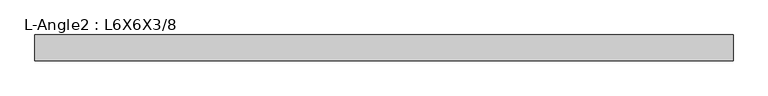
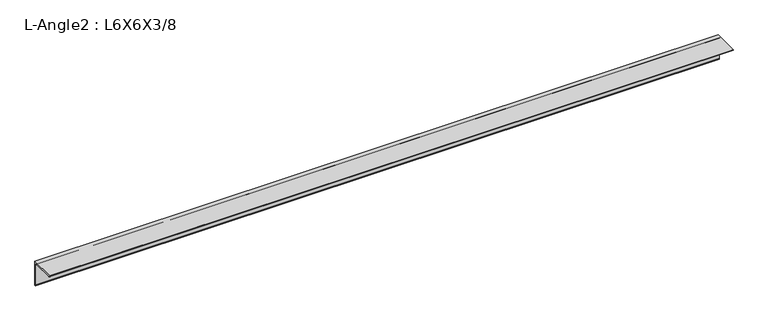
"""IFC4 building model written with IfcOpenShell, lengths in millimetres: member geometry, L-Angle2 : L6X6X3/8."""

from ifc_helpers import new_model, si_unit, point, frame, frame_2d, origin, place, context, project, spatial, polyline, circle_curve, trimmed, segment, composite_curve, outline, extrude, source, transform, mapped, element, save


def l_angle2_l6x6x3_8_670392f0(model_context):
    return source(origin(), model_context, "Body", "SweptSolid", [
        extrude(outline(composite_curve([segment(polyline([(41.148, 41.148), (41.148, -111.252)]), True, "CONTINUOUS"), segment(trimmed(circle_curve(frame_2d((41.148, -101.727)), 9.525), [point((41.148, -111.252))], [point((31.623, -101.727))], False, "CARTESIAN"), True, "CONTINUOUS"), segment(polyline([(31.623, -101.727), (31.623, 22.098)]), True, "CONTINUOUS"), segment(trimmed(circle_curve(frame_2d((22.098, 22.098)), 9.525), [point((31.623, 22.098))], [point((22.098, 31.623))], True, "CARTESIAN"), True, "CONTINUOUS"), segment(polyline([(22.098, 31.623), (-101.727, 31.623)]), True, "CONTINUOUS"), segment(trimmed(circle_curve(frame_2d((-101.727, 41.148)), 9.525), [point((-101.727, 31.623))], [point((-111.252, 41.148))], False, "CARTESIAN"), True, "CONTINUOUS"), segment(polyline([(-111.252, 41.148), (41.148, 41.148)]), True, "CONTINUOUS")], self_intersect=False)), frame((-2053.0970548, 0.0, 0.0), z_axis=(1.0, 0.0, 0.0), x_axis=(0.0, 1.0, 0.0)), (0.0, 0.0, 1.0), 4091.5211794),
    ])


if __name__ == "__main__":
    model = new_model("IFC4")
    model_context = context("Model", 3, world=origin())
    ifc_project = project(units=[si_unit("LENGTHUNIT", "METRE", prefix="MILLI")], contexts=[model_context])
    site = spatial("IfcSite", under=ifc_project)
    building = spatial("IfcBuilding", under=site)
    placement = place(None, origin())
    l_angle2_l6x6x3_8_shape = l_angle2_l6x6x3_8_670392f0(model_context)
    element("IfcMember", 1, ObjectType="L-Angle2 : L6X6X3/8", at=placement, inside=building, context=model_context, shape_type="MappedRepresentation", body=[
        mapped(l_angle2_l6x6x3_8_shape, transform((0.0, 0.0, 0.0), x_axis=(1.0, 0.0, 0.0), y_axis=(0.0, 1.0, 0.0), z_axis=(0.0, 0.0, 1.0))),
    ])
    save(model, "model.ifc")

# Revit data of these elements
# Type "L-Angle2 : L6X6X3/8"
#   Assembly Code = "B10"
#   k = 0' - 0 7/8"
#   W = 14.9
#   Length [instance default] = 5' - 0"
#   b = 0' - 6"
#   d = 0' - 6"
#   t = 0' - 0 3/8"
#   x = 0' - 1.62"
#   y = 0' - 1.62"
#   A = 0.0304167 SF
#   Structural Material [instance default] = Steel ASTM A36
# Element 1 (IfcMember, "L-Angle2 : L6X6X3/8")
#   Materials on its faces: "Steel ASTM A36"
# Materials
#   "Steel ASTM A36": class "Metal", colour RGB 199 199 199, transparency 0, Description = "Structural steel, ASTM A36 Grade B, mill finish", Cost = 0
